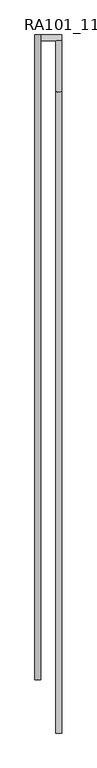
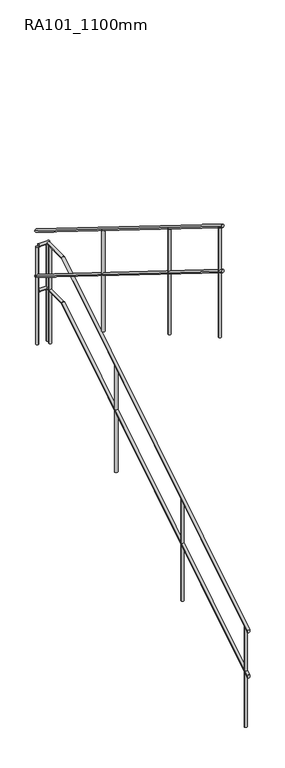
"""IFC4 building model written with IfcOpenShell, lengths in millimetres: railing geometry, RA101_1100mm."""

from ifc_helpers import new_model, si_unit, point, frame, frame_2d, origin, place, context, project, spatial, circle_curve, ellipse_curve, trimmed, segment, composite_curve, outline, extrude, source, transform, mapped, element, save
from ifc_brep_helpers import plane_surface, cylinder_surface, advanced_brep


def ra101_1100mm_1ac2519f(model_context):
    return source(origin(), model_context, "Body", "SolidModel", [
        advanced_brep(
        [(11545.1052251, 14699.5208589, 456.3396197), (11515.1052251, 14699.5208589, 456.3396197), (11545.1052251, 18329.5208589, 2547.0), (11515.1052251, 18329.5208589, 2547.0), (11545.1052251, 18063.8019306, 2547.0), (11515.1052251, 18063.8019306, 2547.0)],
        [
            (0, 1, ellipse_curve(frame((11530.1052251, 14699.5208589, 456.3396197), z_axis=(0.0, -1.0, 0.0), x_axis=(0.0, 0.0, -1.0)), 17.6603803, 15.0)),
            (1, 0, ellipse_curve(frame((11530.1052251, 14699.5208589, 456.3396197), z_axis=(0.0, -1.0, 0.0), x_axis=(0.0, 0.0, -1.0)), 17.6603803, 15.0)),
            (2, 3, circle_curve(frame((11530.1052251, 18329.5208589, 2547.0), z_axis=(0.0, 1.0, 0.0), x_axis=(-1.0, 0.0, 0.0)), 15.0)),
            (3, 2, circle_curve(frame((11530.1052251, 18329.5208589, 2547.0), z_axis=(0.0, 1.0, 0.0), x_axis=(-1.0, 0.0, 0.0)), 15.0)),
            (0, 4),
            (4, 5, ellipse_curve(frame((11530.1052251, 18063.8019306, 2547.0), z_axis=(0.0, -0.9616025257983003, -0.2744459552959912), x_axis=(0.0, 0.2744459552959914, -0.9616025257983002)), 15.5989607, 15.0)),
            (5, 1),
            (5, 4, ellipse_curve(frame((11530.1052251, 18063.8019306, 2547.0), z_axis=(0.0, -0.9616025257983003, -0.2744459552959912), x_axis=(0.0, 0.2744459552959914, -0.9616025257983002)), 15.5989607, 15.0)),
            (4, 2),
            (3, 5),
        ],
        [
            plane_surface(frame((11530.1052251, 14699.5208589, 474.0), z_axis=(0.0, -1.0, 0.0), x_axis=(0.0, 0.0, 1.0))),
            plane_surface(frame((11530.1052251, 18329.5208589, 2562.0), z_axis=(0.0, 1.0, 0.0), x_axis=(0.0, 0.0, 1.0))),
            cylinder_surface(frame((11530.1052251, 14707.4380966, 461.2596175), z_axis=(0.0, -0.8493588352433417, -0.5278158476155052), x_axis=(-1.0, 0.0, 0.0)), 15.0),
            cylinder_surface(frame((11530.1052251, 18059.5208589, 2547.0), z_axis=(0.0, -1.0, 0.0), x_axis=(-1.0, 0.0, 0.0)), 15.0),
        ],
        [
            (0, [[1, 2]]),
            (1, [[3, 4]]),
            (2, [[-1, 5, 6, 7]]),
            (2, [[-2, -7, 8, -5]]),
            (3, [[-6, 9, -4, 10]]),
            (3, [[-8, -10, -3, -9]]),
        ],
    ),
        advanced_brep(
        [(11545.1052251, 18359.5208589, 2547.0), (11545.1052251, 18329.5208589, 2547.0), (11435.1052251, 18359.5208589, 2547.0), (11435.1052251, 18329.5208589, 2547.0)],
        [
            (0, 1, circle_curve(frame((11545.1052251, 18344.5208589, 2547.0), z_axis=(1.0, 0.0, 0.0), x_axis=(0.0, -1.0, 0.0)), 15.0)),
            (1, 0, circle_curve(frame((11545.1052251, 18344.5208589, 2547.0), z_axis=(1.0, 0.0, 0.0), x_axis=(0.0, -1.0, 0.0)), 15.0)),
            (2, 3, circle_curve(frame((11435.1052251, 18344.5208589, 2547.0), z_axis=(-1.0, 0.0, 0.0), x_axis=(0.0, -1.0, 0.0)), 15.0)),
            (3, 2, circle_curve(frame((11435.1052251, 18344.5208589, 2547.0), z_axis=(-1.0, 0.0, 0.0), x_axis=(0.0, -1.0, 0.0)), 15.0)),
            (0, 2),
            (3, 1),
        ],
        [
            plane_surface(frame((11545.1052251, 18344.5208589, 2562.0), z_axis=(1.0, 0.0, 0.0), x_axis=(0.0, -1.0, 0.0))),
            plane_surface(frame((11435.1052251, 18344.5208589, 2562.0), z_axis=(-1.0, 0.0, 0.0), x_axis=(0.0, -1.0, 0.0))),
            cylinder_surface(frame((11545.1052251, 18344.5208589, 2547.0), z_axis=(1.0, 0.0, 0.0), x_axis=(0.0, -1.0, 0.0)), 15.0),
        ],
        [
            (0, [[1, 2]]),
            (1, [[3, 4]]),
            (2, [[-1, 5, -4, 6]]),
            (2, [[-2, -6, -3, -5]]),
        ],
    ),
        advanced_brep(
        [(11405.1052251, 18359.5208589, 2705.9110483), (11435.1052251, 18359.5208589, 2705.9110483), (11405.1052251, 14979.5208589, 4806.3396197), (11435.1052251, 14979.5208589, 4806.3396197)],
        [
            (0, 1, ellipse_curve(frame((11420.1052251, 18359.5208589, 2705.9110483), z_axis=(0.0, 1.0, 0.0), x_axis=(0.0, 0.0, -1.0)), 17.6603803, 15.0)),
            (1, 0, ellipse_curve(frame((11420.1052251, 18359.5208589, 2705.9110483), z_axis=(0.0, 1.0, 0.0), x_axis=(0.0, 0.0, -1.0)), 17.6603803, 15.0)),
            (2, 3, ellipse_curve(frame((11420.1052251, 14979.5208589, 4806.3396197), z_axis=(0.0, -1.0, 0.0), x_axis=(0.0, 0.0, -1.0)), 17.6603803, 15.0)),
            (3, 2, ellipse_curve(frame((11420.1052251, 14979.5208589, 4806.3396197), z_axis=(0.0, -1.0, 0.0), x_axis=(0.0, 0.0, -1.0)), 17.6603803, 15.0)),
            (0, 2),
            (3, 1),
        ],
        [
            plane_surface(frame((11420.1052251, 18359.5208589, 2723.5714286), z_axis=(0.0, 1.0, 0.0), x_axis=(0.0, 0.0, -1.0))),
            plane_surface(frame((11420.1052251, 14979.5208589, 4824.0), z_axis=(0.0, -1.0, 0.0), x_axis=(0.0, 0.0, -1.0))),
            cylinder_surface(frame((11420.1052251, 18351.6036212, 2710.831046), z_axis=(0.0, 0.8493588352433417, -0.5278158476155052), x_axis=(1.0, 0.0, 0.0)), 15.0),
        ],
        [
            (0, [[1, 2]]),
            (1, [[3, 4]]),
            (2, [[-1, 5, -4, 6]]),
            (2, [[-2, -6, -3, -5]]),
        ],
    ),
        advanced_brep(
        [(11545.1052251, 14699.5208589, 956.3396197), (11515.1052251, 14699.5208589, 956.3396197), (11545.1052251, 18063.8019306, 3047.0), (11515.1052251, 18063.8019306, 3047.0), (11545.1052251, 18329.5208589, 3047.0), (11515.1052251, 18329.5208589, 3047.0)],
        [
            (0, 1, ellipse_curve(frame((11530.1052251, 14699.5208589, 956.3396197), z_axis=(0.0, -1.0, 0.0), x_axis=(0.0, 0.0, -1.0)), 17.6603803, 15.0)),
            (1, 0, ellipse_curve(frame((11530.1052251, 14699.5208589, 956.3396197), z_axis=(0.0, -1.0, 0.0), x_axis=(0.0, 0.0, -1.0)), 17.6603803, 15.0)),
            (0, 2),
            (2, 3, ellipse_curve(frame((11530.1052251, 18063.8019306, 3047.0), z_axis=(0.0, -0.9616025257983003, -0.2744459552959912), x_axis=(0.0, 0.2744459552959914, -0.9616025257983002)), 15.5989607, 15.0)),
            (3, 1),
            (3, 2, ellipse_curve(frame((11530.1052251, 18063.8019306, 3047.0), z_axis=(0.0, -0.9616025257983003, -0.2744459552959912), x_axis=(0.0, 0.2744459552959914, -0.9616025257983002)), 15.5989607, 15.0)),
            (4, 5, circle_curve(frame((11530.1052251, 18329.5208589, 3047.0), z_axis=(0.0, 1.0, 0.0), x_axis=(-1.0, 0.0, 0.0)), 15.0)),
            (5, 4, circle_curve(frame((11530.1052251, 18329.5208589, 3047.0), z_axis=(0.0, 1.0, 0.0), x_axis=(-1.0, 0.0, 0.0)), 15.0)),
            (2, 4),
            (5, 3),
        ],
        [
            plane_surface(frame((11530.1052251, 14699.5208589, 974.0), z_axis=(0.0, -1.0, 0.0), x_axis=(0.0, 0.0, 1.0))),
            cylinder_surface(frame((11530.1052251, 14707.4380966, 961.2596175), z_axis=(0.0, -0.8493588352433417, -0.5278158476155052), x_axis=(-1.0, 0.0, 0.0)), 15.0),
            plane_surface(frame((11530.1052251, 18329.5208589, 3062.0), z_axis=(0.0, 1.0, 0.0), x_axis=(0.0, 0.0, 1.0))),
            cylinder_surface(frame((11530.1052251, 18059.5208589, 3047.0), z_axis=(0.0, -1.0, 0.0), x_axis=(-1.0, 0.0, 0.0)), 15.0),
        ],
        [
            (0, [[1, 2]]),
            (1, [[-1, 3, 4, 5]]),
            (1, [[-2, -5, 6, -3]]),
            (2, [[7, 8]]),
            (3, [[-4, 9, -8, 10]]),
            (3, [[-6, -10, -7, -9]]),
        ],
    ),
        advanced_brep(
        [(11545.1052251, 18359.5208589, 3047.0), (11545.1052251, 18329.5208589, 3047.0), (11435.1052251, 18359.5208589, 3047.0), (11435.1052251, 18329.5208589, 3047.0)],
        [
            (0, 1, circle_curve(frame((11545.1052251, 18344.5208589, 3047.0), z_axis=(1.0, 0.0, 0.0), x_axis=(0.0, -1.0, 0.0)), 15.0)),
            (1, 0, circle_curve(frame((11545.1052251, 18344.5208589, 3047.0), z_axis=(1.0, 0.0, 0.0), x_axis=(0.0, -1.0, 0.0)), 15.0)),
            (2, 3, circle_curve(frame((11435.1052251, 18344.5208589, 3047.0), z_axis=(-1.0, 0.0, 0.0), x_axis=(0.0, -1.0, 0.0)), 15.0)),
            (3, 2, circle_curve(frame((11435.1052251, 18344.5208589, 3047.0), z_axis=(-1.0, 0.0, 0.0), x_axis=(0.0, -1.0, 0.0)), 15.0)),
            (0, 2),
            (3, 1),
        ],
        [
            plane_surface(frame((11545.1052251, 18344.5208589, 3062.0), z_axis=(1.0, 0.0, 0.0), x_axis=(0.0, -1.0, 0.0))),
            plane_surface(frame((11435.1052251, 18344.5208589, 3062.0), z_axis=(-1.0, 0.0, 0.0), x_axis=(0.0, -1.0, 0.0))),
            cylinder_surface(frame((11545.1052251, 18344.5208589, 3047.0), z_axis=(1.0, 0.0, 0.0), x_axis=(0.0, -1.0, 0.0)), 15.0),
        ],
        [
            (0, [[1, 2]]),
            (1, [[3, 4]]),
            (2, [[-1, 5, -4, 6]]),
            (2, [[-2, -6, -3, -5]]),
        ],
    ),
        advanced_brep(
        [(11405.1052251, 18359.5208589, 3205.9110483), (11435.1052251, 18359.5208589, 3205.9110483), (11405.1052251, 14979.5208589, 5306.3396197), (11435.1052251, 14979.5208589, 5306.3396197)],
        [
            (0, 1, ellipse_curve(frame((11420.1052251, 18359.5208589, 3205.9110483), z_axis=(0.0, 1.0, 0.0), x_axis=(0.0, 0.0, -1.0)), 17.6603803, 15.0)),
            (1, 0, ellipse_curve(frame((11420.1052251, 18359.5208589, 3205.9110483), z_axis=(0.0, 1.0, 0.0), x_axis=(0.0, 0.0, -1.0)), 17.6603803, 15.0)),
            (2, 3, ellipse_curve(frame((11420.1052251, 14979.5208589, 5306.3396197), z_axis=(0.0, -1.0, 0.0), x_axis=(0.0, 0.0, -1.0)), 17.6603803, 15.0)),
            (3, 2, ellipse_curve(frame((11420.1052251, 14979.5208589, 5306.3396197), z_axis=(0.0, -1.0, 0.0), x_axis=(0.0, 0.0, -1.0)), 17.6603803, 15.0)),
            (0, 2),
            (3, 1),
        ],
        [
            plane_surface(frame((11420.1052251, 18359.5208589, 3223.5714286), z_axis=(0.0, 1.0, 0.0), x_axis=(0.0, 0.0, -1.0))),
            plane_surface(frame((11420.1052251, 14979.5208589, 5324.0), z_axis=(0.0, -1.0, 0.0), x_axis=(0.0, 0.0, -1.0))),
            cylinder_surface(frame((11420.1052251, 18351.6036212, 3210.831046), z_axis=(0.0, 0.8493588352433417, -0.5278158476155052), x_axis=(1.0, 0.0, 0.0)), 15.0),
        ],
        [
            (0, [[1, 2]]),
            (1, [[3, 4]]),
            (2, [[-1, 5, -4, 6]]),
            (2, [[-2, -6, -3, -5]]),
        ],
    ),
        extrude(outline(composite_curve([segment(trimmed(circle_curve(frame_2d((11420.1052251, 15944.5208589)), 15.0), [point((11435.1052251, 15944.5208589))], [point((11405.1052251, 15944.5208589))], False, "CARTESIAN"), True, "CONTINUOUS"), segment(trimmed(circle_curve(frame_2d((11420.1052251, 15944.5208589)), 15.0), [point((11405.1052251, 15944.5208589))], [point((11435.1052251, 15944.5208589))], False, "CARTESIAN"), True, "CONTINUOUS")], self_intersect=False)), frame((0.0, 0.0, 3528.0), z_axis=(0.0, 0.0, 1.0), x_axis=(1.0, 0.0, 0.0)), (0.0, 0.0, 1.0), 1166.3214286),
        extrude(outline(composite_curve([segment(trimmed(circle_curve(frame_2d((11420.1052251, 17144.5208589)), 15.0), [point((11435.1052251, 17144.5208589))], [point((11405.1052251, 17144.5208589))], False, "CARTESIAN"), True, "CONTINUOUS"), segment(trimmed(circle_curve(frame_2d((11420.1052251, 17144.5208589)), 15.0), [point((11405.1052251, 17144.5208589))], [point((11435.1052251, 17144.5208589))], False, "CARTESIAN"), True, "CONTINUOUS")], self_intersect=False)), frame((0.0, 0.0, 2832.0), z_axis=(0.0, 0.0, 1.0), x_axis=(1.0, 0.0, 0.0)), (0.0, 0.0, 1.0), 1116.6071429),
        extrude(outline(composite_curve([segment(trimmed(circle_curve(frame_2d((11530.1052251, 18299.5208589)), 15.0), [point((11515.1052251, 18299.5208589))], [point((11545.1052251, 18299.5208589))], False, "CARTESIAN"), True, "CONTINUOUS"), segment(trimmed(circle_curve(frame_2d((11530.1052251, 18299.5208589)), 15.0), [point((11545.1052251, 18299.5208589))], [point((11515.1052251, 18299.5208589))], False, "CARTESIAN"), True, "CONTINUOUS")], self_intersect=False)), frame((0.0, 0.0, 1962.0), z_axis=(0.0, 0.0, 1.0), x_axis=(1.0, 0.0, 0.0)), (0.0, 0.0, 1.0), 1070.0),
        extrude(outline(composite_curve([segment(trimmed(circle_curve(frame_2d((11530.1052251, 17099.5208589)), 15.0), [point((11515.1052251, 17099.5208589))], [point((11545.1052251, 17099.5208589))], False, "CARTESIAN"), True, "CONTINUOUS"), segment(trimmed(circle_curve(frame_2d((11530.1052251, 17099.5208589)), 15.0), [point((11545.1052251, 17099.5208589))], [point((11515.1052251, 17099.5208589))], False, "CARTESIAN"), True, "CONTINUOUS")], self_intersect=False)), frame((0.0, 0.0, 1266.0), z_axis=(0.0, 0.0, 1.0), x_axis=(1.0, 0.0, 0.0)), (0.0, 0.0, 1.0), 1169.4285714),
        extrude(outline(composite_curve([segment(trimmed(circle_curve(frame_2d((11530.1052251, 15899.5208589)), 15.0), [point((11515.1052251, 15899.5208589))], [point((11545.1052251, 15899.5208589))], False, "CARTESIAN"), True, "CONTINUOUS"), segment(trimmed(circle_curve(frame_2d((11530.1052251, 15899.5208589)), 15.0), [point((11545.1052251, 15899.5208589))], [point((11515.1052251, 15899.5208589))], False, "CARTESIAN"), True, "CONTINUOUS")], self_intersect=False)), frame((0.0, 0.0, 570.0), z_axis=(0.0, 0.0, 1.0), x_axis=(1.0, 0.0, 0.0)), (0.0, 0.0, 1.0), 1119.7142857),
        extrude(outline(composite_curve([segment(trimmed(circle_curve(frame_2d((11420.1052251, 18344.5208589)), 15.0), [point((11420.1052251, 18329.5208589))], [point((11420.1052251, 18359.5208589))], False, "CARTESIAN"), True, "CONTINUOUS"), segment(trimmed(circle_curve(frame_2d((11420.1052251, 18344.5208589)), 15.0), [point((11420.1052251, 18359.5208589))], [point((11420.1052251, 18329.5208589))], False, "CARTESIAN"), True, "CONTINUOUS")], self_intersect=False)), frame((0.0, 0.0, 1962.0), z_axis=(0.0, 0.0, 1.0), x_axis=(1.0, 0.0, 0.0)), (0.0, 0.0, 1.0), 1070.0),
        extrude(outline(composite_curve([segment(trimmed(circle_curve(frame_2d((11530.1052251, 18344.5208589)), 15.0), [point((11515.1052251, 18344.5208589))], [point((11545.1052251, 18344.5208589))], False, "CARTESIAN"), True, "CONTINUOUS"), segment(trimmed(circle_curve(frame_2d((11530.1052251, 18344.5208589)), 15.0), [point((11545.1052251, 18344.5208589))], [point((11515.1052251, 18344.5208589))], False, "CARTESIAN"), True, "CONTINUOUS")], self_intersect=False)), frame((0.0, 0.0, 1962.0), z_axis=(0.0, 0.0, 1.0), x_axis=(1.0, 0.0, 0.0)), (0.0, 0.0, 1.0), 1070.0),
        extrude(outline(composite_curve([segment(trimmed(circle_curve(frame_2d((11420.1052251, 15029.5208589)), 15.0), [point((11435.1052251, 15029.5208589))], [point((11405.1052251, 15029.5208589))], False, "CARTESIAN"), True, "CONTINUOUS"), segment(trimmed(circle_curve(frame_2d((11420.1052251, 15029.5208589)), 15.0), [point((11405.1052251, 15029.5208589))], [point((11435.1052251, 15029.5208589))], False, "CARTESIAN"), True, "CONTINUOUS")], self_intersect=False)), frame((0.0, 0.0, 4050.0), z_axis=(0.0, 0.0, 1.0), x_axis=(1.0, 0.0, 0.0)), (0.0, 0.0, 1.0), 1212.9285714),
        extrude(outline(composite_curve([segment(trimmed(circle_curve(frame_2d((11530.1052251, 14749.5208589)), 15.0), [point((11515.1052251, 14749.5208589))], [point((11545.1052251, 14749.5208589))], False, "CARTESIAN"), True, "CONTINUOUS"), segment(trimmed(circle_curve(frame_2d((11530.1052251, 14749.5208589)), 15.0), [point((11545.1052251, 14749.5208589))], [point((11515.1052251, 14749.5208589))], False, "CARTESIAN"), True, "CONTINUOUS")], self_intersect=False)), frame((0.0, 0.0, -126.0), z_axis=(0.0, 0.0, 1.0), x_axis=(1.0, 0.0, 0.0)), (0.0, 0.0, 1.0), 1101.0714286),
    ])


if __name__ == "__main__":
    model = new_model("IFC4")
    model_context = context("Model", 3, world=origin())
    ifc_project = project(units=[si_unit("LENGTHUNIT", "METRE", prefix="MILLI")], contexts=[model_context])
    site = spatial("IfcSite", under=ifc_project)
    building = spatial("IfcBuilding", under=site)
    placement = place(None, origin())
    ra101_1100mm_shape = ra101_1100mm_1ac2519f(model_context)
    element("IfcRailing", 1, ObjectType="RA101_1100mm", at=placement, inside=building, context=model_context, shape_type="MappedRepresentation", body=[
        mapped(ra101_1100mm_shape, transform((0.0, 0.0, 0.0), x_axis=(1.0, 0.0, 0.0), y_axis=(0.0, 1.0, 0.0), z_axis=(0.0, 0.0, 1.0))),
    ])
    save(model, "model.ifc")
